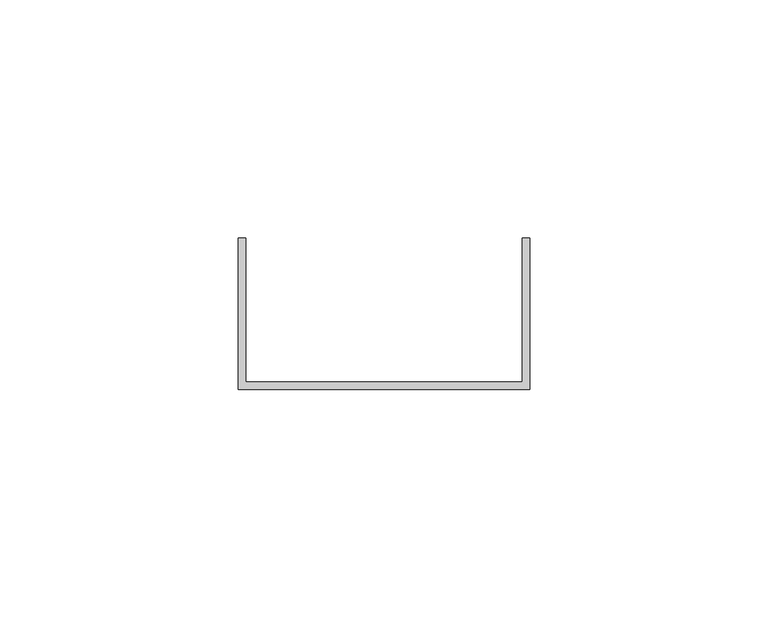
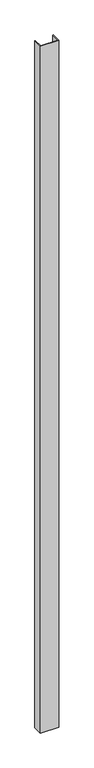
"""IFC4 building model written with IfcOpenShell, lengths in millimetres: proxy geometry, Generic Models 7:Generic Models 1:3:Generic Models 1:3 : Generic Models 7:Generic Models 1:305549:3:Generic Models 1:3:Generic Models 1:3 : Generic Models 7:Generic Models 1:305549:3 : Generic Models 7:Generic Models 1:3:Generic Models 1:3 : Generic Models 7:Generic Models 1:305549:301244:10 : Generic Models 7:Generic Models 1:3:Generic Models 1:3 : Generic Models 7:Generic Models 1:305549:3:Generic Models 1:3:Generic Models 1:3 : Generic Models 7:Generic Models 1:305549:3 : Generic Models 7:Generic Models 1:3:Generic Models 1:3 : Generic Models 7:Generic Models 1:305549:301244:308848."""

from ifc_helpers import new_model, si_unit, frame, origin, place, context, project, spatial, polyline, outline, extrude, source, transform, mapped, element, save


def generic_models_ab168dd0(model_context):
    return source(origin(), model_context, "Body", "SweptSolid", [
        extrude(outline(polyline([(579322.7929739, -579013.3913841), (579322.7929739, -578981.6413841), (579324.3804739, -578981.6413841), (579324.3804739, -579011.8038841), (579382.3242239, -579011.8038841), (579382.3242239, -578981.6413841), (579383.9117239, -578981.6413841), (579383.9117239, -579013.3913841), (579322.7929739, -579013.3913841)])), frame((0.0, 0.0, 3721.1), z_axis=(0.0, 0.0, 1.0), x_axis=(1.0, 0.0, 0.0)), (0.0, 0.0, 1.0), 2430.9324376),
    ])


if __name__ == "__main__":
    model = new_model("IFC4")
    model_context = context("Model", 3, world=origin())
    ifc_project = project(units=[si_unit("LENGTHUNIT", "METRE", prefix="MILLI")], contexts=[model_context])
    site = spatial("IfcSite", under=ifc_project)
    building = spatial("IfcBuilding", under=site)
    placement = place(None, origin())
    generic_models_shape = generic_models_ab168dd0(model_context)
    element("IfcBuildingElementProxy", 1, Name="Generic Models 7:Generic Models 1:3:Generic Models 1:3 : Generic Models 7:Generic Models 1:305549:3:Generic Models 1:3:Generic Models 1:3 : Generic Models 7:Generic Models 1:305549:3 : Generic Models 7:Generic Models 1:3:Generic Models 1:3 : Generic Models 7:Generic Models 1:305549:301244:10 : Generic Models 7:Generic Models 1:3:Generic Models 1:3 : Generic Models 7:Generic Models 1:305549:3:Generic Models 1:3:Generic Models 1:3 : Generic Models 7:Generic Models 1:305549:3 : Generic Models 7:Generic Models 1:3:Generic Models 1:3 : Generic Models 7:Generic Models 1:305549:301244:308848", ObjectType="Generic Models 7:Generic Models 1:3:Generic Models 1:3 : Generic Models 7:Generic Models 1:305549:3:Generic Models 1:3:Generic Models 1:3 : Generic Models 7:Generic Models 1:305549:3 : Generic Models 7:Generic Models 1:3:Generic Models 1:3 : Generic Models 7:Generic Models 1:305549:301244:10 : Generic Models 7:Generic Models 1:3:Generic Models 1:3 : Generic Models 7:Generic Models 1:305549:3:Generic Models 1:3:Generic Models 1:3 : Generic Models 7:Generic Models 1:305549:3 : Generic Models 7:Generic Models 1:3:Generic Models 1:3 : Generic Models 7:Generic Models 1:305549:301244:308848", at=placement, inside=building, context=model_context, shape_type="MappedRepresentation", body=[
        mapped(generic_models_shape, transform((0.0, 0.0, 0.0), x_axis=(1.0, 0.0, 0.0), y_axis=(0.0, 1.0, 0.0), z_axis=(0.0, 0.0, 1.0))),
    ])
    save(model, "model.ifc")

# Revit data of these elements
# Type "Generic Models 7:Generic Models 1:3:Generic Models 1:3 : Generic Models 7:Generic Models 1:305549:3:Generic Models 1:3:Generic Models 1:3 : Generic Models 7:Generic Models 1:305549:3 : Generic Models 7:Generic Models 1:3:Generic Models 1:3 : Generic Models 7:Generic Models 1:305549:301244:10 : Generic Models 7:Generic Models 1:3:Generic Models 1:3 : Generic Models 7:Generic Models 1:305549:3:Generic Models 1:3:Generic Models 1:3 : Generic Models 7:Generic Models 1:305549:3 : Generic Models 7:Generic Models 1:3:Generic Models 1:3 : Generic Models 7:Generic Models 1:305549:301244:308848"
#   NameOverride = "Generic Models 7:Generic Models 1:3:Generic Models 1:3 : Generic Models 7:Generic Models 1:305549:3:Generic Models 1:3:Generic Models 1:3 : Generic Models 7:Generic Models 1:305549:3 : Generic Models 7:Generic Models 1:3:Generic Models 1:3 : Generic Models 7:Generic Models 1:305549:301244:308848"
#   ObjectTypeOverride = "Generic Models 1:3:Generic Models 1:3 : Generic Models 7:Generic Models 1:305549:3 : Generic Models 7:Generic Models 1:3:Generic Models 1:3 : Generic Models 7:Generic Models 1:305549:301244"
#   Reference = "Generic Models 1"
#   Tag = "308848"
# Element 1 (IfcBuildingElementProxy, "Generic Models 7:Generic Models 1:3:Generic Models 1:3 : Generic Models 7:Generic Models 1:305549:3:Generic Models 1:3:Generic Models 1:3 : Generic Models 7:Generic Models 1:305549:3 : Generic Models 7:Generic Models 1:3:Generic Models 1:3 : Generic Models 7:Generic Models 1:305549:301244:10 : Generic Models 7:Generic Models 1:3:Generic Models 1:3 : Generic Models 7:Generic Models 1:305549:3:Generic Models 1:3:Generic Models 1:3 : Generic Models 7:Generic Models 1:305549:3 : Generic Models 7:Generic Models 1:3:Generic Models 1:3 : Generic Models 7:Generic Models 1:305549:301244:308848")
#   Materials on its faces: "GALVANIZED U-CHANNEL (250T125-33)"
# Materials
#   "GALVANIZED U-CHANNEL (250T125-33)": class "Unassigned", colour RGB 202 201 200, transparency 0, Keynote = "M05451300.02", Cost = 0
